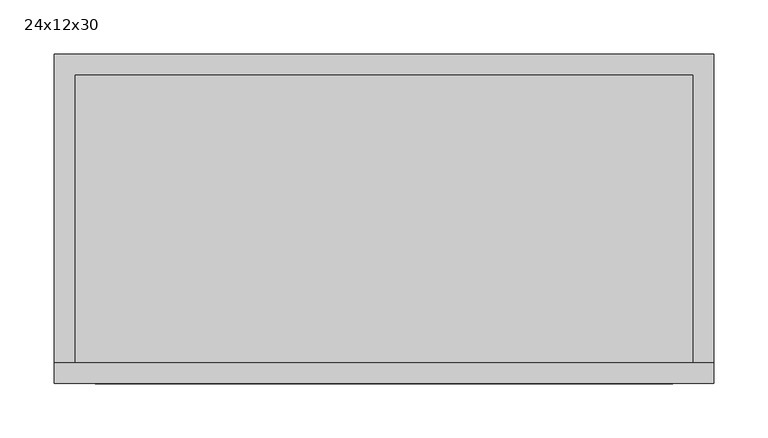
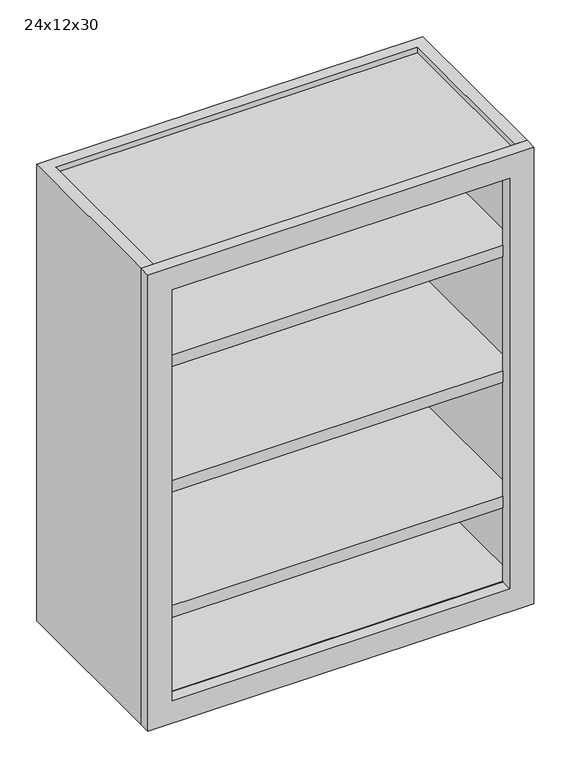
"""IFC4 building model written with IfcOpenShell, lengths in millimetres: furniture geometry, Bookcase-Merillat : 24x12x30."""

from ifc_helpers import new_model, si_unit, frame, origin, place, context, project, spatial, polyline, outline, extrude, faceted_brep, source, transform, mapped, element, save


def furniture_24x12x30_d5dca78b(model_context):
    return source(origin(), model_context, "Body", "SolidModel", [
        extrude(outline(polyline([(-285.75, 133.35), (285.75, 133.35), (285.75, -133.35), (-285.75, -133.35), (-285.75, 133.35)])), frame((0.0, 0.0, 161.925), z_axis=(0.0, 0.0, 1.0), x_axis=(1.0, 0.0, 0.0)), (0.0, 0.0, 1.0), 19.3909952),
        extrude(outline(polyline([(-285.75, 133.35), (285.75, 133.35), (285.75, -133.35), (-285.75, -133.35), (-285.75, 133.35)])), frame((0.0, 0.0, 580.6840048), z_axis=(0.0, 0.0, 1.0), x_axis=(1.0, 0.0, 0.0)), (0.0, 0.0, 1.0), 19.3909952),
        extrude(outline(polyline([(-285.75, 133.35), (285.75, 133.35), (285.75, -133.35), (-285.75, -133.35), (-285.75, 133.35)])), frame((0.0, 0.0, 371.3180074), z_axis=(0.0, 0.0, 1.0), x_axis=(1.0, 0.0, 0.0)), (0.0, 0.0, 1.0), 19.3909952),
        extrude(outline(polyline([(-285.75, 133.35), (285.75, 133.35), (285.75, -133.35), (-285.75, -133.35), (-285.75, 133.35)])), frame((0.0, 0.0, 19.3909952), z_axis=(0.0, 0.0, 1.0), x_axis=(1.0, 0.0, 0.0)), (0.0, 0.0, 1.0), 19.3909952),
        extrude(outline(polyline([(0.0, -304.8), (0.0, 304.8), (762.0, 304.8), (762.0, -304.8), (0.0, -304.8)]), holes=[polyline([(723.9, -266.7), (723.9, 266.7), (38.1, 266.7), (38.1, -266.7), (723.9, -266.7)])]), frame((0.0, -152.4, 0.0), z_axis=(0.0, 1.0, 0.0), x_axis=(0.0, 0.0, 1.0)), (0.0, 0.0, 1.0), 19.05),
        faceted_brep([(-285.75, -133.35, 19.3909952), (285.75, -133.35, 19.3909952), (285.75, 133.35, 19.3909952), (-285.75, 133.35, 19.3909952), (-304.8, 152.4, 0.0), (304.8, 152.4, 0.0), (304.8, -133.35, 0.0), (-304.8, -133.35, 0.0), (-304.8, -133.35, 762.0), (304.8, -133.35, 762.0), (285.75, -133.35, 762.0), (285.75, -133.35, 752.7909423), (-285.75, -133.35, 752.7909423), (-285.75, -133.35, 762.0), (-285.75, -133.35, 742.6090048), (285.75, -133.35, 742.6090048), (-285.75, 133.35, 752.7909423), (285.75, 133.35, 752.7909423), (-285.75, 133.35, 762.0), (285.75, 133.35, 762.0), (-304.8, 152.4, 762.0), (304.8, 152.4, 762.0), (-285.75, 133.35, 742.6090048), (285.75, 133.35, 742.6090048)], [[[0, 1, 2, 3]], [[4, 5, 6, 7]], [[8, 7, 6, 9, 10, 11, 12, 13], [1, 0, 14, 15]], [[16, 12, 11, 17]], [[12, 16, 18, 13]], [[17, 11, 10, 19]], [[16, 17, 19, 18]], [[20, 8, 13, 18, 19, 10, 9, 21]], [[8, 20, 4, 7]], [[0, 3, 22, 14]], [[3, 2, 23, 22]], [[2, 1, 15, 23]], [[21, 9, 6, 5]], [[20, 21, 5, 4]], [[15, 14, 22, 23]]]),
    ])


if __name__ == "__main__":
    model = new_model("IFC4")
    model_context = context("Model", 3, world=origin())
    ifc_project = project(units=[si_unit("LENGTHUNIT", "METRE", prefix="MILLI")], contexts=[model_context])
    site = spatial("IfcSite", under=ifc_project)
    building = spatial("IfcBuilding", under=site)
    placement = place(None, origin())
    furniture_24x12x30_shape = furniture_24x12x30_d5dca78b(model_context)
    element("IfcFurniture", 1, ObjectType="Bookcase-Merillat : 24x12x30", at=placement, inside=building, context=model_context, shape_type="MappedRepresentation", body=[
        mapped(furniture_24x12x30_shape, transform((0.0, 0.0, 0.0), x_axis=(1.0, 0.0, 0.0), y_axis=(0.0, 1.0, 0.0), z_axis=(0.0, 0.0, 1.0))),
    ])
    save(model, "model.ifc")

# Revit data of these elements
# Type "Bookcase-Merillat : 24x12x30"
#   URL = "https://www.merillat.com/"
#   Product Page URL = "https://www.merillat.com/our-products/"
#   Product Documentation Link = "http://merillatbusiness.com/wp-content/uploads/2014/07/Merillat_Classic_Catalog.pdf"
#   Model = "BK1848"
#   Manufacturer = "Merillat"
#   Description = "Bookcase"
#   Construction Type = "Bookcase"
#   Assembly Code = "E2020200"
#   Width = 2' - 0"
#   Shelving Height = 0' - 6 3/4"
#   Height = 2' - 6"
#   Depth = 1' - 0"
#   Default Elevation = 4' - 0"
#   Cabinet Shell = 0' - 0 3/4"
#   COBie.Type = no
#   Two Drawer = yes
#   Shelves Bookcase = yes
#   Number of Shelves = 3
#   No Shelf Bookcase = no
#   Middle Shelf = yes
#   Shelving Material = Wood - Merillat - Hazelnut
#   Bookcase Material = Wood - Merillat - Hazelnut
# Element 1 (IfcFurniture, "Bookcase-Merillat : 24x12x30")
#   Materials on its faces: "Wood - Merillat - Hazelnut"
# Materials
#   "Wood - Merillat - Hazelnut": class "Wood", colour RGB 138 103 81, transparency 0, Cost = 0
